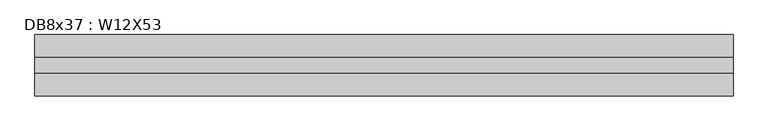
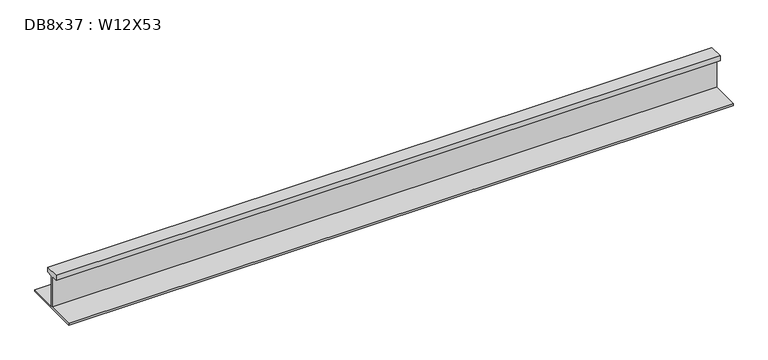
"""IFC4 building model written with IfcOpenShell, lengths in millimetres: beam geometry, DB8x37 : W12X53."""

from ifc_helpers import new_model, si_unit, frame, origin, place, context, project, spatial, polyline, outline, extrude, source, transform, mapped, element, save


def db8x37_w12x53_1d0335d4(model_context):
    return source(origin(), model_context, "Body", "SweptSolid", [
        extrude(outline(polyline([(38.1, 145.415), (38.1, 120.015), (2.921, 120.015), (2.921, -48.4505), (152.4, -48.4505), (152.4, -58.1025), (-152.4, -58.1025), (-152.4, -48.4505), (-2.921, -48.4505), (-2.921, 120.015), (-38.1, 120.015), (-38.1, 145.415), (38.1, 145.415)])), frame((-1713.23, 0.0, 0.0), z_axis=(1.0, 0.0, 0.0), x_axis=(0.0, 1.0, 0.0)), (0.0, 0.0, 1.0), 3456.559),
    ])


if __name__ == "__main__":
    model = new_model("IFC4")
    model_context = context("Model", 3, world=origin())
    ifc_project = project(units=[si_unit("LENGTHUNIT", "METRE", prefix="MILLI")], contexts=[model_context])
    site = spatial("IfcSite", under=ifc_project)
    building = spatial("IfcBuilding", under=site)
    placement = place(None, origin())
    db8x37_w12x53_shape = db8x37_w12x53_1d0335d4(model_context)
    element("IfcBeam", 1, ObjectType="DB8x37 : W12X53", at=placement, inside=building, context=model_context, shape_type="MappedRepresentation", body=[
        mapped(db8x37_w12x53_shape, transform((0.0, 0.0, 0.0), x_axis=(1.0, 0.0, 0.0), y_axis=(0.0, 1.0, 0.0), z_axis=(0.0, 0.0, 1.0))),
    ])
    save(model, "model.ifc")

# Revit data of these elements
# Type "DB8x37 : W12X53"
#   Assembly Code = "B10"
#   W = 53
#   Length [instance default] = 5' - 0"
#   bf = 0' - 10"
#   d = 1' - 0.1"
#   k = 0' - 1 3/8"
#   k2 = 0' - 0.8"
#   tf = 0' - 0.575"
#   tw = 0' - 0.345"
#   A = 0.108333 SF
#   Structural Material [instance default] = Steel ASTM A992
# Element 1 (IfcBeam, "DB8x37 : W12X53")
#   Materials on its faces: "Steel ASTM A992"
# Materials
#   "Steel ASTM A992": class "Metal", colour RGB 199 199 199, transparency 0, Description = "Structural steel 50ksi", Cost = 0
